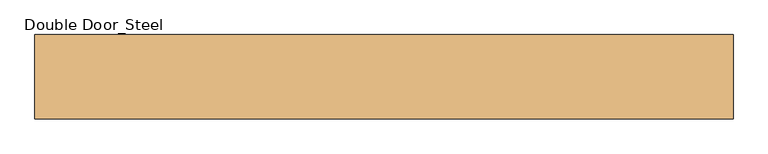
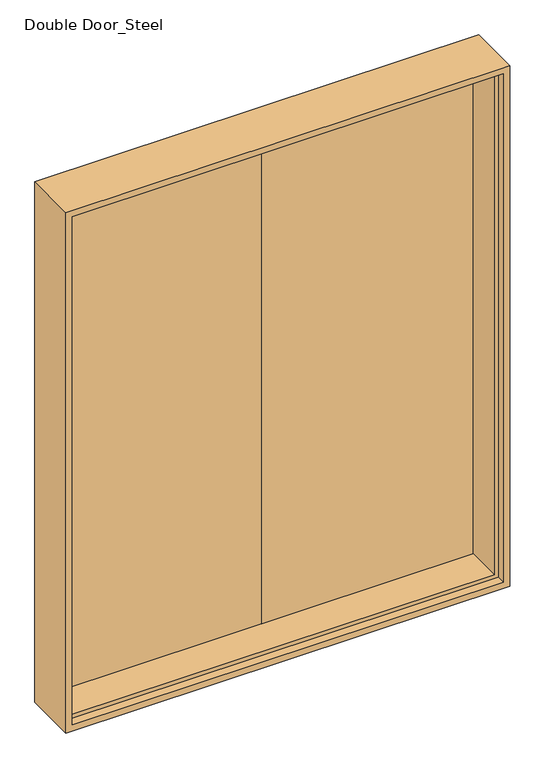
"""IFC4 building model written with IfcOpenShell, lengths in millimetres: door geometry, Double Door_Steel : H_DR_AR B12_Door_Double_W2100xH2580_No FR_SD-5."""

import ifcopenshell
import ifcopenshell.guid

model = None  # the IFC model being written
_history = None  # IfcOwnerHistory: only IFC2X3 demands one
_inside = {}  # id of a spatial element -> (the spatial element, [elements in it])
_under = {}  # id of a project, library or spatial element -> (it, [spatial elements below it])
_declared = {}  # id of a project -> (the project, [libraries it declares])
_typed = {}  # id of a type object -> (the type object, [elements of that type])
_made_of = {}  # id of a material, layer set ... -> (it, [elements and type objects made of it])


def new_model(schema):
    """Start an empty IFC model of exactly this schema.

    Asked for "IFC4X3", IfcOpenShell would pick the latest addendum, in which some entities
    have other attributes; the version numbers below select the first issue.
    IFC2X3 requires an IfcOwnerHistory on every rooted entity: one is made here for all.
    """
    global model, _history
    if schema == "IFC4X3":
        model = ifcopenshell.file(schema_version=(4, 3, 0, 0))
    else:
        model = ifcopenshell.file(schema=schema)
    _inside.clear()
    _under.clear()
    _declared.clear()
    _typed.clear()
    _made_of.clear()
    _history = None
    if model.schema == "IFC2X3":
        org = make("IfcOrganization", Name="unknown")
        user = make(
            "IfcPersonAndOrganization",
            ThePerson=make("IfcPerson", FamilyName="unknown"),
            TheOrganization=org,
        )
        app = make(
            "IfcApplication",
            ApplicationDeveloper=org,
            Version="unknown",
            ApplicationFullName="unknown",
            ApplicationIdentifier="unknown",
        )
        _history = make(
            "IfcOwnerHistory",
            OwningUser=user,
            OwningApplication=app,
            ChangeAction="ADDED",
            CreationDate=0,
        )
    return model


def make(cls, **values):
    """One entity of the class cls with the attributes given. An attribute that is None is left unset."""
    return model.create_entity(
        cls, **{name: value for name, value in values.items() if value is not None}
    )


def rooted(cls, **values):
    """An entity with a GlobalId (a new one), such as an element, a storey or a relation."""
    return make(cls, GlobalId=ifcopenshell.guid.new(), OwnerHistory=_history, **values)


def si_unit(unit_type, name, prefix=None):
    """IfcSIUnit, for example si_unit("LENGTHUNIT", "METRE", prefix="MILLI")."""
    return make("IfcSIUnit", UnitType=unit_type, Prefix=prefix, Name=name)


def assignment(units):
    """IfcUnitAssignment: the units of a project."""
    return None if units is None else make("IfcUnitAssignment", Units=units)


def point(xyz):
    """IfcCartesianPoint."""
    return None if xyz is None else make("IfcCartesianPoint", Coordinates=xyz)


def direction(xyz):
    """IfcDirection."""
    return None if xyz is None else make("IfcDirection", DirectionRatios=xyz)


def frame(location, z_axis=None, x_axis=None):
    """IfcAxis2Placement3D, a coordinate frame: its origin and axes. An axis left out is left unset."""
    return make(
        "IfcAxis2Placement3D",
        Location=point(location),
        Axis=direction(z_axis),
        RefDirection=direction(x_axis),
    )


def origin():
    """The frame at (0, 0, 0) with its axes left unset."""
    return frame((0.0, 0.0, 0.0))


def place(relative_to, where):
    """IfcLocalPlacement: puts the frame where relative to a parent placement (None: the world)."""
    return make(
        "IfcLocalPlacement", PlacementRelTo=relative_to, RelativePlacement=where
    )


def context(
    kind, dimensions, precision=None, world=None, true_north=None, identifier=None
):
    """IfcGeometricRepresentationContext, for example the 3D "Model" context."""
    return make(
        "IfcGeometricRepresentationContext",
        ContextIdentifier=identifier,
        ContextType=kind,
        CoordinateSpaceDimension=dimensions,
        Precision=precision,
        WorldCoordinateSystem=world,
        TrueNorth=true_north,
    )


def project(units=None, contexts=None):
    """IfcProject with its units and contexts."""
    return rooted(
        "IfcProject",
        Name="project",
        RepresentationContexts=contexts,
        UnitsInContext=assignment(units),
    )


def spatial(cls, under=None, at=None, **own):
    """A site, building, storey or space (cls), placed at a placement, below another one or the project."""
    s = rooted(cls, ObjectPlacement=at, **own)
    if under is not None:
        _under.setdefault(under.id(), (under, []))[1].append(s)
    return s


def polyline(points):
    """IfcPolyline through the points."""
    return make("IfcPolyline", Points=[point(p) for p in points])


def outline(outer, holes=None, kind="AREA"):
    """IfcArbitraryClosedProfileDef: a profile drawn as a closed curve; with holes, ...WithVoids."""
    if holes is None:
        return make("IfcArbitraryClosedProfileDef", ProfileType=kind, OuterCurve=outer)
    return make(
        "IfcArbitraryProfileDefWithVoids",
        ProfileType=kind,
        OuterCurve=outer,
        InnerCurves=holes,
    )


def extrude(swept, where, along, depth):
    """IfcExtrudedAreaSolid: the profile swept, set in the frame where, extruded along a direction by depth."""
    return make(
        "IfcExtrudedAreaSolid",
        SweptArea=swept,
        Position=where,
        ExtrudedDirection=direction(along),
        Depth=depth,
    )


def faces_of(points, faces, orient=None, outer=None):
    """IfcFace entities. A face is a list of loops; a loop is a list of indices into points, from 0.

    orient and outer hold one flag for each loop. By default every Orientation is true, the
    first loop of a face is its IfcFaceOuterBound and the others are IfcFaceBound.
    """
    made = []
    for i, loops in enumerate(faces):
        bounds = []
        for j, loop in enumerate(loops):
            is_outer = j == 0 if outer is None else outer[i][j]
            bounds.append(
                make(
                    "IfcFaceOuterBound" if is_outer else "IfcFaceBound",
                    Bound=make("IfcPolyLoop", Polygon=[points[k] for k in loop]),
                    Orientation=True if orient is None else orient[i][j],
                )
            )
        made.append(make("IfcFace", Bounds=bounds))
    return made


def faceted_brep(points, faces, orient=None, outer=None, voids=None):
    """IfcFacetedBrep: a solid bounded by flat faces; with voids (closed shells), ...WithVoids."""
    shared = [point(p) for p in points]
    hull = make("IfcClosedShell", CfsFaces=faces_of(shared, faces, orient, outer))
    if voids is None:
        return make("IfcFacetedBrep", Outer=hull)
    return make(
        "IfcFacetedBrepWithVoids",
        Outer=hull,
        Voids=[
            make(cls, CfsFaces=faces_of(shared, fs, o, b)) for cls, fs, o, b in voids
        ],
    )


def shape(context_of_items, identifier, shape_type, items):
    """IfcShapeRepresentation: the items that make up one representation, for example the "Body"."""
    return make(
        "IfcShapeRepresentation",
        ContextOfItems=context_of_items,
        RepresentationIdentifier=identifier,
        RepresentationType=shape_type,
        Items=items,
    )


def source(mapping_origin, context_of_items, identifier, shape_type, items):
    """IfcRepresentationMap: a shape defined once, which mapped items show again and again."""
    return make(
        "IfcRepresentationMap",
        MappingOrigin=mapping_origin,
        MappedRepresentation=shape(context_of_items, identifier, shape_type, items),
    )


def transform(
    local_origin,
    x_axis=None,
    y_axis=None,
    z_axis=None,
    scale=None,
    scale2=None,
    scale3=None,
    uniform=True,
):
    """IfcCartesianTransformationOperator3D, or its non-uniform kind. x_axis, y_axis, z_axis: its Axis1, 2, 3."""
    if uniform:
        return make(
            "IfcCartesianTransformationOperator3D",
            Axis1=direction(x_axis),
            Axis2=direction(y_axis),
            LocalOrigin=point(local_origin),
            Scale=scale,
            Axis3=direction(z_axis),
        )
    return make(
        "IfcCartesianTransformationOperator3DnonUniform",
        Axis1=direction(x_axis),
        Axis2=direction(y_axis),
        LocalOrigin=point(local_origin),
        Scale=scale,
        Axis3=direction(z_axis),
        Scale2=scale2,
        Scale3=scale3,
    )


def mapped(mapping_source, mapping_target):
    """IfcMappedItem: shows the shape of a source again, moved by a transform."""
    return make(
        "IfcMappedItem", MappingSource=mapping_source, MappingTarget=mapping_target
    )


def made_of(thing, what):
    """Note that an element or type object is made of a material, layer set ...; save() writes the relation."""
    if what is not None:
        _made_of.setdefault(what.id(), (what, []))[1].append(thing)
    return thing


def element(
    cls,
    number,
    at=None,
    inside=None,
    cuts=None,
    type_object=None,
    material=None,
    context=None,
    identifier="Body",
    shape_type=None,
    held_by="IfcProductDefinitionShape",
    body=None,
    shapes=None,
    **own,
):
    """One element of the class cls, such as IfcWall. Its Tag is "e" and its number.

    at: its placement. inside: the storey or other place that contains it. cuts: it is an
    opening in that element (IfcRelVoidsElement). A single representation is given by context,
    identifier, shape_type and body (its items); several are given by shapes. held_by: the class
    of the entity that holds the representations. save() writes the other relations.
    """
    e = rooted(cls, Tag="e%d" % number, ObjectPlacement=at, **own)
    if body is not None:
        shapes = [shape(context, identifier, shape_type, body)]
    if shapes is not None:
        e.Representation = make(held_by, Representations=shapes)
    if inside is not None:
        _inside.setdefault(inside.id(), (inside, []))[1].append(e)
    if cuts is not None:
        rooted(
            "IfcRelVoidsElement", RelatingBuildingElement=cuts, RelatedOpeningElement=e
        )
    if type_object is not None:
        _typed.setdefault(type_object.id(), (type_object, []))[1].append(e)
    return made_of(e, material)


def aggregate(whole, parts):
    """IfcRelAggregates: a whole, such as a stair, and the parts it consists of."""
    return rooted("IfcRelAggregates", RelatingObject=whole, RelatedObjects=parts)


def save(model, path):
    """Write the relations noted so far, then the file.

    IfcRelAggregates (storeys below a building ...), IfcRelContainedInSpatialStructure (elements
    in a storey), IfcRelDefinesByType, IfcRelAssociatesMaterial and IfcRelDeclares: one each for
    every whole, place, type object, material and project.
    """
    for whole, parts in _under.values():
        aggregate(whole, parts)
    for where, things in _inside.values():
        rooted(
            "IfcRelContainedInSpatialStructure",
            RelatedElements=things,
            RelatingStructure=where,
        )
    for kind, things in _typed.values():
        rooted("IfcRelDefinesByType", RelatedObjects=things, RelatingType=kind)
    for what, things in _made_of.values():
        rooted("IfcRelAssociatesMaterial", RelatedObjects=things, RelatingMaterial=what)
    for by, libraries in _declared.values():
        rooted("IfcRelDeclares", RelatingContext=by, RelatedDefinitions=libraries)
    model.write(path)


def double_door_steel_c24d22a6(model_context):
    return source(origin(), model_context, "Body", "SolidModel", [
        faceted_brep([(-1035.0, -125.0, 2565.0), (-1035.0, 125.0, 2565.0), (-1035.0, 125.0, 0.0), (-1035.0, -125.0, 0.0), (1035.0, 125.0, 0.0), (1035.0, 125.0, 2565.0), (1005.0, 125.0, 2535.0), (-1005.0, 125.0, 2535.0), (-1005.0, 125.0, 30.0), (1005.0, 125.0, 30.0), (1035.0, -125.0, 0.0), (1035.0, -125.0, 2565.0), (1005.0, -125.0, 30.0), (-1005.0, -125.0, 30.0), (-1005.0, -125.0, 2535.0), (1005.0, -125.0, 2535.0), (-1005.0, -85.0, 2535.0), (-1005.0, -85.0, 30.0), (1005.0, -85.0, 30.0), (1005.0, -85.0, 2535.0), (985.0, -85.0, 2515.0), (985.0, -85.0, 50.0), (-985.0, -85.0, 50.0), (-985.0, -85.0, 2515.0), (-985.0, 85.0, 2515.0), (-985.0, 85.0, 50.0), (985.0, 85.0, 50.0), (1005.0, 85.0, 30.0), (-1005.0, 85.0, 30.0), (-1005.0, 85.0, 2535.0), (1005.0, 85.0, 2535.0), (985.0, 85.0, 2515.0)], [[[0, 1, 2, 3]], [[4, 2, 1, 5], [6, 7, 8, 9]], [[3, 2, 4, 10]], [[11, 0, 3, 10], [12, 13, 14, 15]], [[16, 14, 13, 17]], [[17, 13, 12, 18]], [[16, 17, 18, 19], [20, 21, 22, 23]], [[24, 23, 22, 25]], [[25, 22, 21, 26]], [[27, 28, 29, 30], [31, 24, 25, 26]], [[7, 29, 28, 8]], [[8, 28, 27, 9]], [[10, 4, 5, 11]], [[9, 27, 30, 6]], [[18, 12, 15, 19]], [[26, 21, 20, 31]], [[11, 5, 1, 0]], [[19, 15, 14, 16]], [[31, 20, 23, 24]], [[6, 30, 29, 7]]]),
        extrude(outline(polyline([(1005.0, 85.0), (0.0, 85.0), (0.0, 125.0), (1005.0, 125.0), (1005.0, 85.0)])), frame((0.0, 0.0, 30.0), z_axis=(0.0, 0.0, 1.0), x_axis=(1.0, 0.0, 0.0)), (0.0, 0.0, 1.0), 2505.0),
        extrude(outline(polyline([(0.0, 85.0), (-1005.0, 85.0), (-1005.0, 125.0), (0.0, 125.0), (0.0, 85.0)])), frame((0.0, 0.0, 30.0), z_axis=(0.0, 0.0, 1.0), x_axis=(1.0, 0.0, 0.0)), (0.0, 0.0, 1.0), 2505.0),
    ])


if __name__ == "__main__":
    model = new_model("IFC4")
    model_context = context("Model", 3, world=origin())
    ifc_project = project(units=[si_unit("LENGTHUNIT", "METRE", prefix="MILLI")], contexts=[model_context])
    site = spatial("IfcSite", under=ifc_project)
    building = spatial("IfcBuilding", under=site)
    placement = place(None, origin())
    double_door_steel_shape = double_door_steel_c24d22a6(model_context)
    element("IfcDoor", 1, ObjectType="Double Door_Steel : H_DR_AR B12_Door_Double_W2100xH2580_No FR_SD-5", at=placement, inside=building, context=model_context, shape_type="MappedRepresentation", body=[
        mapped(double_door_steel_shape, transform((0.0, 0.0, 0.0), x_axis=(1.0, 0.0, 0.0), y_axis=(0.0, 1.0, 0.0), z_axis=(0.0, 0.0, 1.0))),
    ])
    save(model, "model.ifc")

# Revit data of these elements
# Type "Double Door_Steel : H_DR_AR B12_Door_Double_W2100xH2580_No FR_SD-5"
#   Type Mark = "444"
#   프레임 = ""
#   철물 = ""
#   유리/마감 = ""
#   위치/개소 = ""
#   부호 = ""
#   문번호 = ""
#   문기호 = "SD-5"
#   Analytic Construction = "<None>"
#   Door Width = 1005 mm
#   Height = 2580 mm
#   Width = 2100 mm
#   Define Thermal Properties by = 1
#   문 틀 = none
#   문 = none
#   Function = (empty or 0)
#   Assembly Code = ""
#   Wall Closure = (empty or 0)
